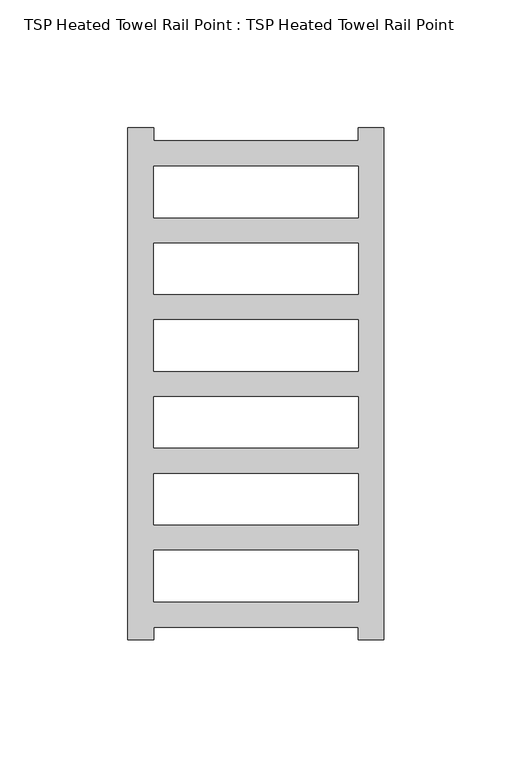
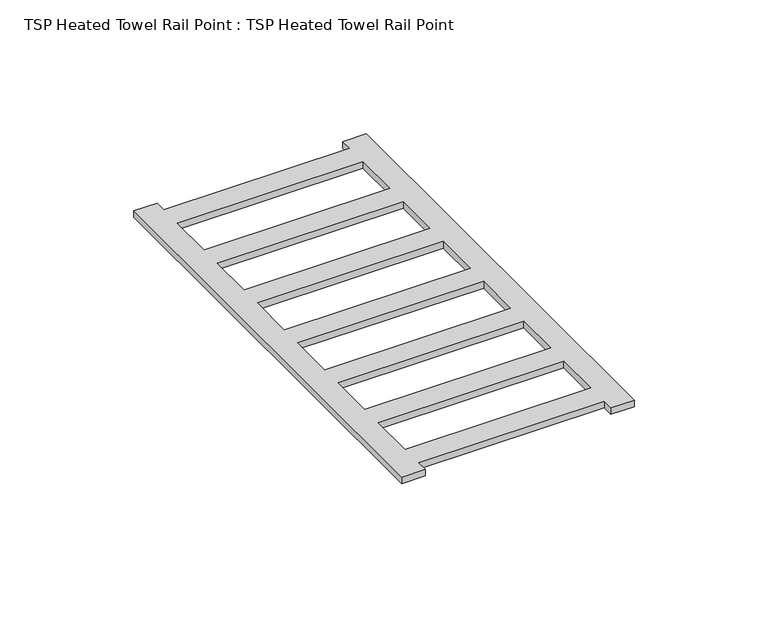
"""IFC4 building model written with IfcOpenShell, lengths in millimetres: proxy geometry, TSP Heated Towel Rail Point : TSP Heated Towel Rail Point."""

from ifc_helpers import new_model, si_unit, origin, origin_with_axes, place, context, project, spatial, polyline, outline, extrude, source, transform, mapped, element, save


def tsp_heated_towel_rail_point_tsp_heated_towel_rail_point_6a43df22(model_context):
    return source(origin(), model_context, "Body", "SweptSolid", [
        extrude(outline(polyline([(-10.0, 100.0), (0.0, 100.0), (0.0, -100.0), (-10.0, -100.0), (-10.0, -95.0), (-90.0, -95.0), (-90.0, -100.0), (-100.0, -100.0), (-100.0, 100.0), (-90.0, 100.0), (-90.0, 95.0), (-10.0, 95.0), (-10.0, 100.0)]), holes=[polyline([(-10.0, 5.0), (-10.0, 25.0), (-90.0, 25.0), (-90.0, 5.0), (-10.0, 5.0)]), polyline([(-90.0, -5.0), (-90.0, -25.0), (-10.0, -25.0), (-10.0, -5.0), (-90.0, -5.0)]), polyline([(-10.0, 35.0), (-10.0, 55.0), (-90.0, 55.0), (-90.0, 35.0), (-10.0, 35.0)]), polyline([(-10.0, 65.0), (-10.0, 85.0), (-90.0, 85.0), (-90.0, 65.0), (-10.0, 65.0)]), polyline([(-10.0, -35.0), (-90.0, -35.0), (-90.0, -55.0), (-10.0, -55.0), (-10.0, -35.0)]), polyline([(-10.0, -65.0), (-90.0, -65.0), (-90.0, -85.0), (-10.0, -85.0), (-10.0, -65.0)])]), origin_with_axes(), (0.0, 0.0, 1.0), 3.0),
    ])


if __name__ == "__main__":
    model = new_model("IFC4")
    model_context = context("Model", 3, world=origin())
    ifc_project = project(units=[si_unit("LENGTHUNIT", "METRE", prefix="MILLI")], contexts=[model_context])
    site = spatial("IfcSite", under=ifc_project)
    building = spatial("IfcBuilding", under=site)
    placement = place(None, origin())
    tsp_heated_towel_rail_point_tsp_heated_towel_rail_point_shape = tsp_heated_towel_rail_point_tsp_heated_towel_rail_point_6a43df22(model_context)
    element("IfcBuildingElementProxy", 1, Name="TSP Heated Towel Rail Point : TSP Heated Towel Rail Point", ObjectType="TSP Heated Towel Rail Point : TSP Heated Towel Rail Point", at=placement, inside=building, context=model_context, shape_type="MappedRepresentation", body=[
        mapped(tsp_heated_towel_rail_point_tsp_heated_towel_rail_point_shape, transform((0.0, 0.0, 0.0), x_axis=(1.0, 0.0, 0.0), y_axis=(0.0, 1.0, 0.0), z_axis=(0.0, 0.0, 1.0))),
    ])
    save(model, "model.ifc")

# Revit data of these elements
# Type "TSP Heated Towel Rail Point : TSP Heated Towel Rail Point"
#   Model = "TSP_ELECHTR"
#   Default Elevation = 0
# Element 1 (IfcBuildingElementProxy, "TSP Heated Towel Rail Point : TSP Heated Towel Rail Point")
#   Materials on its faces: "Plastic, Opaque Black"
# Materials
#   "Plastic, Opaque Black": class "Plastic", colour RGB 0 0 0, transparency 0.7, Description = "Plastic, generic, opaque black", Cost = 0
